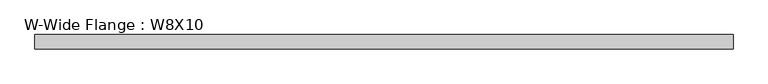
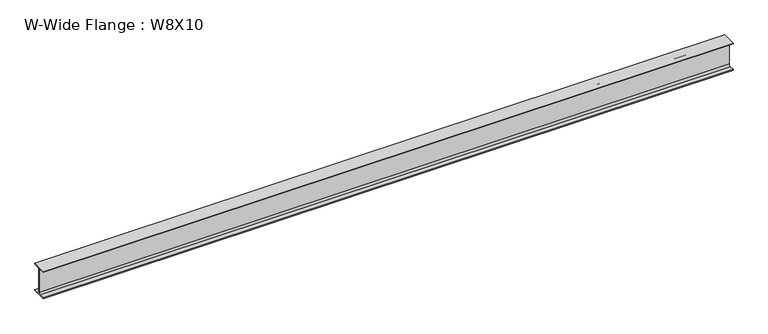
"""IFC4 building model written with IfcOpenShell, lengths in millimetres: beam geometry, W-Wide Flange : W8X10."""

from ifc_helpers import new_model, si_unit, point, frame, frame_2d, origin, place, context, project, spatial, polyline, circle_curve, trimmed, segment, composite_curve, outline, extrude, source, transform, mapped, element, save


def w_wide_flange_w8x10_84c81e36(model_context):
    return source(origin(), model_context, "Body", "SweptSolid", [
        extrude(outline(composite_curve([segment(polyline([(50.038, -94.996), (50.038, -100.203), (-50.038, -100.203), (-50.038, -94.996), (-14.4145, -94.996)]), True, "CONTINUOUS"), segment(trimmed(circle_curve(frame_2d((-14.4145, -82.7405)), 12.2555), [point((-14.4145, -94.996))], [point((-2.159, -82.7405))], True, "CARTESIAN"), True, "CONTINUOUS"), segment(polyline([(-2.159, -82.7405), (-2.159, 82.7405)]), True, "CONTINUOUS"), segment(trimmed(circle_curve(frame_2d((-14.4145, 82.7405)), 12.2555), [point((-2.159, 82.7405))], [point((-14.4145, 94.996))], True, "CARTESIAN"), True, "CONTINUOUS"), segment(polyline([(-14.4145, 94.996), (-50.038, 94.996), (-50.038, 100.203), (50.038, 100.203), (50.038, 94.996), (14.4145, 94.996)]), True, "CONTINUOUS"), segment(trimmed(circle_curve(frame_2d((14.4145, 82.7405)), 12.2555), [point((14.4145, 94.996))], [point((2.159, 82.7405))], True, "CARTESIAN"), True, "CONTINUOUS"), segment(polyline([(2.159, 82.7405), (2.159, -82.7405)]), True, "CONTINUOUS"), segment(trimmed(circle_curve(frame_2d((14.4145, -82.7405)), 12.2555), [point((2.159, -82.7405))], [point((14.4145, -94.996))], True, "CARTESIAN"), True, "CONTINUOUS"), segment(polyline([(14.4145, -94.996), (50.038, -94.996)]), True, "CONTINUOUS")], self_intersect=False)), frame((-2413.8255, 0.0, 0.0), z_axis=(1.0, 0.0, 0.0), x_axis=(0.0, 1.0, 0.0)), (0.0, 0.0, 1.0), 4837.938),
    ])


if __name__ == "__main__":
    model = new_model("IFC4")
    model_context = context("Model", 3, world=origin())
    ifc_project = project(units=[si_unit("LENGTHUNIT", "METRE", prefix="MILLI")], contexts=[model_context])
    site = spatial("IfcSite", under=ifc_project)
    building = spatial("IfcBuilding", under=site)
    placement = place(None, origin())
    w_wide_flange_w8x10_shape = w_wide_flange_w8x10_84c81e36(model_context)
    element("IfcBeam", 1, ObjectType="W-Wide Flange : W8X10", at=placement, inside=building, context=model_context, shape_type="MappedRepresentation", body=[
        mapped(w_wide_flange_w8x10_shape, transform((0.0, 0.0, 0.0), x_axis=(1.0, 0.0, 0.0), y_axis=(0.0, 1.0, 0.0), z_axis=(0.0, 0.0, 1.0))),
    ])
    save(model, "model.ifc")

# Revit data of these elements
# Type "W-Wide Flange : W8X10"
#   Assembly Code = "B10"
#   W = 10
#   Length [instance default] = 1524 mm
#   bf = 100.076 mm
#   d = 200.406 mm
#   k = 17.463 mm
#   k2 = 12.255 mm
#   tf = 5.207 mm
#   tw = 4.318 mm
#   A = 0.00190967 m²
#   Structural Material [instance default] = Steel ASTM A992
# Element 1 (IfcBeam, "W-Wide Flange : W8X10")
#   Structural Material = Aluminum, Anodized Red
#   Materials on its faces: "Aluminum, Anodized Red"
# Materials
#   "Steel ASTM A992": class "Metal", colour RGB 128 0 0, transparency 0, Description = "Structural steel 50ksi", Cost = 0
#   "Aluminum, Anodized Red": class "Metal", colour RGB 120 120 120, transparency 0, Description = "Anodized aluminum, red", Cost = 0
